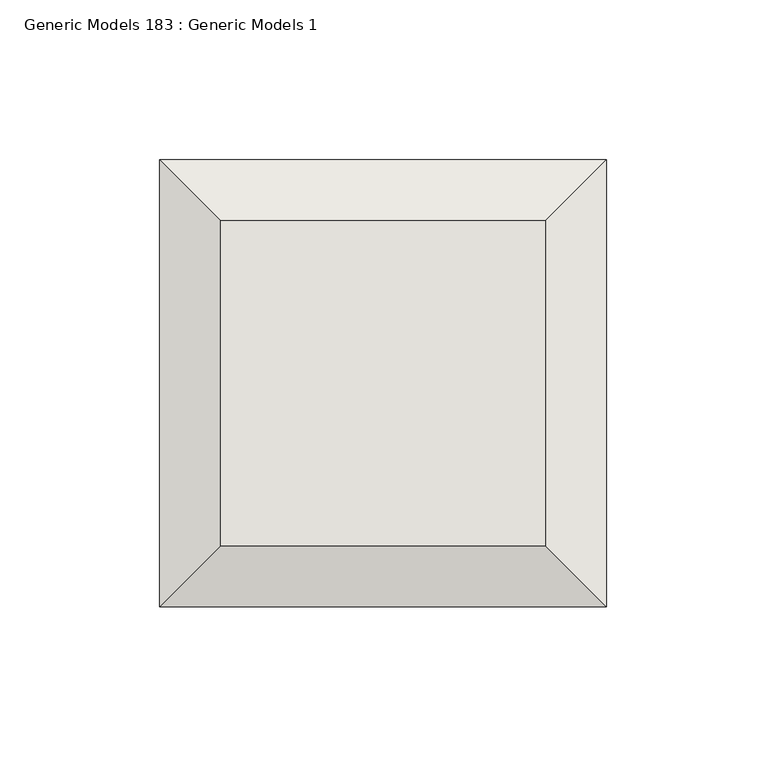
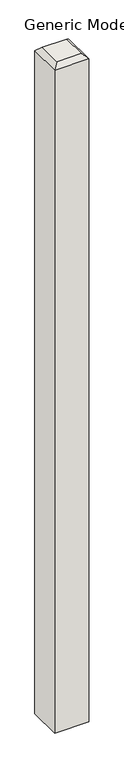
"""IFC4 building model written with IfcOpenShell, lengths in millimetres: wall geometry, Generic Models 183 : Generic Models 1."""

import ifcopenshell
import ifcopenshell.guid

model = None  # the IFC model being written
_history = None  # IfcOwnerHistory: only IFC2X3 demands one
_inside = {}  # id of a spatial element -> (the spatial element, [elements in it])
_under = {}  # id of a project, library or spatial element -> (it, [spatial elements below it])
_declared = {}  # id of a project -> (the project, [libraries it declares])
_typed = {}  # id of a type object -> (the type object, [elements of that type])
_made_of = {}  # id of a material, layer set ... -> (it, [elements and type objects made of it])


def new_model(schema):
    """Start an empty IFC model of exactly this schema.

    Asked for "IFC4X3", IfcOpenShell would pick the latest addendum, in which some entities
    have other attributes; the version numbers below select the first issue.
    IFC2X3 requires an IfcOwnerHistory on every rooted entity: one is made here for all.
    """
    global model, _history
    if schema == "IFC4X3":
        model = ifcopenshell.file(schema_version=(4, 3, 0, 0))
    else:
        model = ifcopenshell.file(schema=schema)
    _inside.clear()
    _under.clear()
    _declared.clear()
    _typed.clear()
    _made_of.clear()
    _history = None
    if model.schema == "IFC2X3":
        org = make("IfcOrganization", Name="unknown")
        user = make(
            "IfcPersonAndOrganization",
            ThePerson=make("IfcPerson", FamilyName="unknown"),
            TheOrganization=org,
        )
        app = make(
            "IfcApplication",
            ApplicationDeveloper=org,
            Version="unknown",
            ApplicationFullName="unknown",
            ApplicationIdentifier="unknown",
        )
        _history = make(
            "IfcOwnerHistory",
            OwningUser=user,
            OwningApplication=app,
            ChangeAction="ADDED",
            CreationDate=0,
        )
    return model


def make(cls, **values):
    """One entity of the class cls with the attributes given. An attribute that is None is left unset."""
    return model.create_entity(
        cls, **{name: value for name, value in values.items() if value is not None}
    )


def rooted(cls, **values):
    """An entity with a GlobalId (a new one), such as an element, a storey or a relation."""
    return make(cls, GlobalId=ifcopenshell.guid.new(), OwnerHistory=_history, **values)


def si_unit(unit_type, name, prefix=None):
    """IfcSIUnit, for example si_unit("LENGTHUNIT", "METRE", prefix="MILLI")."""
    return make("IfcSIUnit", UnitType=unit_type, Prefix=prefix, Name=name)


def assignment(units):
    """IfcUnitAssignment: the units of a project."""
    return None if units is None else make("IfcUnitAssignment", Units=units)


def point(xyz):
    """IfcCartesianPoint."""
    return None if xyz is None else make("IfcCartesianPoint", Coordinates=xyz)


def direction(xyz):
    """IfcDirection."""
    return None if xyz is None else make("IfcDirection", DirectionRatios=xyz)


def frame(location, z_axis=None, x_axis=None):
    """IfcAxis2Placement3D, a coordinate frame: its origin and axes. An axis left out is left unset."""
    return make(
        "IfcAxis2Placement3D",
        Location=point(location),
        Axis=direction(z_axis),
        RefDirection=direction(x_axis),
    )


def origin():
    """The frame at (0, 0, 0) with its axes left unset."""
    return frame((0.0, 0.0, 0.0))


def place(relative_to, where):
    """IfcLocalPlacement: puts the frame where relative to a parent placement (None: the world)."""
    return make(
        "IfcLocalPlacement", PlacementRelTo=relative_to, RelativePlacement=where
    )


def context(
    kind, dimensions, precision=None, world=None, true_north=None, identifier=None
):
    """IfcGeometricRepresentationContext, for example the 3D "Model" context."""
    return make(
        "IfcGeometricRepresentationContext",
        ContextIdentifier=identifier,
        ContextType=kind,
        CoordinateSpaceDimension=dimensions,
        Precision=precision,
        WorldCoordinateSystem=world,
        TrueNorth=true_north,
    )


def project(units=None, contexts=None):
    """IfcProject with its units and contexts."""
    return rooted(
        "IfcProject",
        Name="project",
        RepresentationContexts=contexts,
        UnitsInContext=assignment(units),
    )


def spatial(cls, under=None, at=None, **own):
    """A site, building, storey or space (cls), placed at a placement, below another one or the project."""
    s = rooted(cls, ObjectPlacement=at, **own)
    if under is not None:
        _under.setdefault(under.id(), (under, []))[1].append(s)
    return s


def faces_of(points, faces, orient=None, outer=None):
    """IfcFace entities. A face is a list of loops; a loop is a list of indices into points, from 0.

    orient and outer hold one flag for each loop. By default every Orientation is true, the
    first loop of a face is its IfcFaceOuterBound and the others are IfcFaceBound.
    """
    made = []
    for i, loops in enumerate(faces):
        bounds = []
        for j, loop in enumerate(loops):
            is_outer = j == 0 if outer is None else outer[i][j]
            bounds.append(
                make(
                    "IfcFaceOuterBound" if is_outer else "IfcFaceBound",
                    Bound=make("IfcPolyLoop", Polygon=[points[k] for k in loop]),
                    Orientation=True if orient is None else orient[i][j],
                )
            )
        made.append(make("IfcFace", Bounds=bounds))
    return made


def faceted_brep(points, faces, orient=None, outer=None, voids=None):
    """IfcFacetedBrep: a solid bounded by flat faces; with voids (closed shells), ...WithVoids."""
    shared = [point(p) for p in points]
    hull = make("IfcClosedShell", CfsFaces=faces_of(shared, faces, orient, outer))
    if voids is None:
        return make("IfcFacetedBrep", Outer=hull)
    return make(
        "IfcFacetedBrepWithVoids",
        Outer=hull,
        Voids=[
            make(cls, CfsFaces=faces_of(shared, fs, o, b)) for cls, fs, o, b in voids
        ],
    )


def shape(context_of_items, identifier, shape_type, items):
    """IfcShapeRepresentation: the items that make up one representation, for example the "Body"."""
    return make(
        "IfcShapeRepresentation",
        ContextOfItems=context_of_items,
        RepresentationIdentifier=identifier,
        RepresentationType=shape_type,
        Items=items,
    )


def source(mapping_origin, context_of_items, identifier, shape_type, items):
    """IfcRepresentationMap: a shape defined once, which mapped items show again and again."""
    return make(
        "IfcRepresentationMap",
        MappingOrigin=mapping_origin,
        MappedRepresentation=shape(context_of_items, identifier, shape_type, items),
    )


def transform(
    local_origin,
    x_axis=None,
    y_axis=None,
    z_axis=None,
    scale=None,
    scale2=None,
    scale3=None,
    uniform=True,
):
    """IfcCartesianTransformationOperator3D, or its non-uniform kind. x_axis, y_axis, z_axis: its Axis1, 2, 3."""
    if uniform:
        return make(
            "IfcCartesianTransformationOperator3D",
            Axis1=direction(x_axis),
            Axis2=direction(y_axis),
            LocalOrigin=point(local_origin),
            Scale=scale,
            Axis3=direction(z_axis),
        )
    return make(
        "IfcCartesianTransformationOperator3DnonUniform",
        Axis1=direction(x_axis),
        Axis2=direction(y_axis),
        LocalOrigin=point(local_origin),
        Scale=scale,
        Axis3=direction(z_axis),
        Scale2=scale2,
        Scale3=scale3,
    )


def mapped(mapping_source, mapping_target):
    """IfcMappedItem: shows the shape of a source again, moved by a transform."""
    return make(
        "IfcMappedItem", MappingSource=mapping_source, MappingTarget=mapping_target
    )


def made_of(thing, what):
    """Note that an element or type object is made of a material, layer set ...; save() writes the relation."""
    if what is not None:
        _made_of.setdefault(what.id(), (what, []))[1].append(thing)
    return thing


def element(
    cls,
    number,
    at=None,
    inside=None,
    cuts=None,
    type_object=None,
    material=None,
    context=None,
    identifier="Body",
    shape_type=None,
    held_by="IfcProductDefinitionShape",
    body=None,
    shapes=None,
    **own,
):
    """One element of the class cls, such as IfcWall. Its Tag is "e" and its number.

    at: its placement. inside: the storey or other place that contains it. cuts: it is an
    opening in that element (IfcRelVoidsElement). A single representation is given by context,
    identifier, shape_type and body (its items); several are given by shapes. held_by: the class
    of the entity that holds the representations. save() writes the other relations.
    """
    e = rooted(cls, Tag="e%d" % number, ObjectPlacement=at, **own)
    if body is not None:
        shapes = [shape(context, identifier, shape_type, body)]
    if shapes is not None:
        e.Representation = make(held_by, Representations=shapes)
    if inside is not None:
        _inside.setdefault(inside.id(), (inside, []))[1].append(e)
    if cuts is not None:
        rooted(
            "IfcRelVoidsElement", RelatingBuildingElement=cuts, RelatedOpeningElement=e
        )
    if type_object is not None:
        _typed.setdefault(type_object.id(), (type_object, []))[1].append(e)
    return made_of(e, material)


def aggregate(whole, parts):
    """IfcRelAggregates: a whole, such as a stair, and the parts it consists of."""
    return rooted("IfcRelAggregates", RelatingObject=whole, RelatedObjects=parts)


def save(model, path):
    """Write the relations noted so far, then the file.

    IfcRelAggregates (storeys below a building ...), IfcRelContainedInSpatialStructure (elements
    in a storey), IfcRelDefinesByType, IfcRelAssociatesMaterial and IfcRelDeclares: one each for
    every whole, place, type object, material and project.
    """
    for whole, parts in _under.values():
        aggregate(whole, parts)
    for where, things in _inside.values():
        rooted(
            "IfcRelContainedInSpatialStructure",
            RelatedElements=things,
            RelatingStructure=where,
        )
    for kind, things in _typed.values():
        rooted("IfcRelDefinesByType", RelatedObjects=things, RelatingType=kind)
    for what, things in _made_of.values():
        rooted("IfcRelAssociatesMaterial", RelatedObjects=things, RelatingMaterial=what)
    for by, libraries in _declared.values():
        rooted("IfcRelDeclares", RelatingContext=by, RelatedDefinitions=libraries)
    model.write(path)


def generic_models_183_generic_models_1_4255d89c(model_context):
    return source(origin(), model_context, "Body", "Brep", [
        faceted_brep([(54227.4125, 528.6375, -1066.8), (54087.7125, 528.6375, -1066.8), (54087.7125, 528.6375, 1809.75), (54227.4125, 528.6375, 1809.75), (54227.4125, 388.9375, -1066.8), (54227.4125, 388.9375, 1809.75), (54087.7125, 388.9375, 1809.75), (54087.7125, 388.9375, -1066.8), (54106.7625, 407.9875, 1828.8), (54208.3625, 407.9875, 1828.8), (54208.3625, 509.5875, 1828.8), (54106.7625, 509.5875, 1828.8)], [[[0, 1, 2, 3]], [[4, 5, 6, 7]], [[1, 0, 4, 7]], [[2, 1, 7, 6]], [[8, 9, 10, 11]], [[0, 3, 5, 4]], [[2, 6, 8, 11]], [[5, 3, 10, 9]], [[6, 5, 9, 8]], [[3, 2, 11, 10]]]),
    ])


if __name__ == "__main__":
    model = new_model("IFC4")
    model_context = context("Model", 3, world=origin())
    ifc_project = project(units=[si_unit("LENGTHUNIT", "METRE", prefix="MILLI")], contexts=[model_context])
    site = spatial("IfcSite", under=ifc_project)
    building = spatial("IfcBuilding", under=site)
    placement = place(None, origin())
    generic_models_183_generic_models_1_shape = generic_models_183_generic_models_1_4255d89c(model_context)
    element("IfcWall", 1, ObjectType="Generic Models 183 : Generic Models 1", at=placement, inside=building, context=model_context, shape_type="MappedRepresentation", body=[
        mapped(generic_models_183_generic_models_1_shape, transform((0.0, 0.0, 0.0), x_axis=(1.0, 0.0, 0.0), y_axis=(0.0, 1.0, 0.0), z_axis=(0.0, 0.0, 1.0))),
    ])
    save(model, "model.ifc")

# Revit data of these elements
# Element 1 (IfcWall, "Generic Models 183 : Generic Models 1")
#   Materials on its faces: "TREATED 6X6 POST"
# Materials
#   "TREATED 6X6 POST": class "Wood", colour RGB 234 198 147, transparency 0, Description = "Pinus Echinata", Cost = 0
